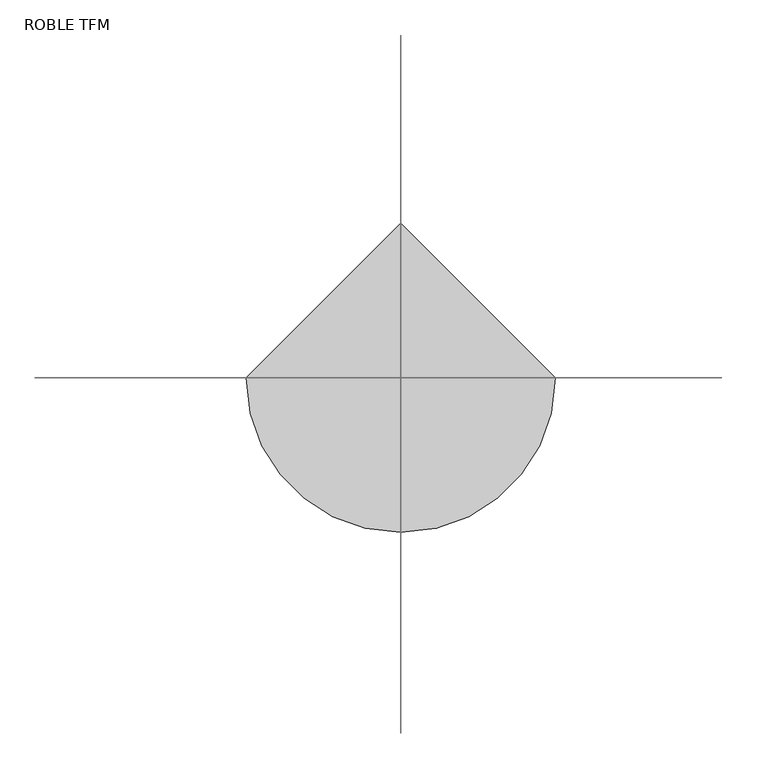
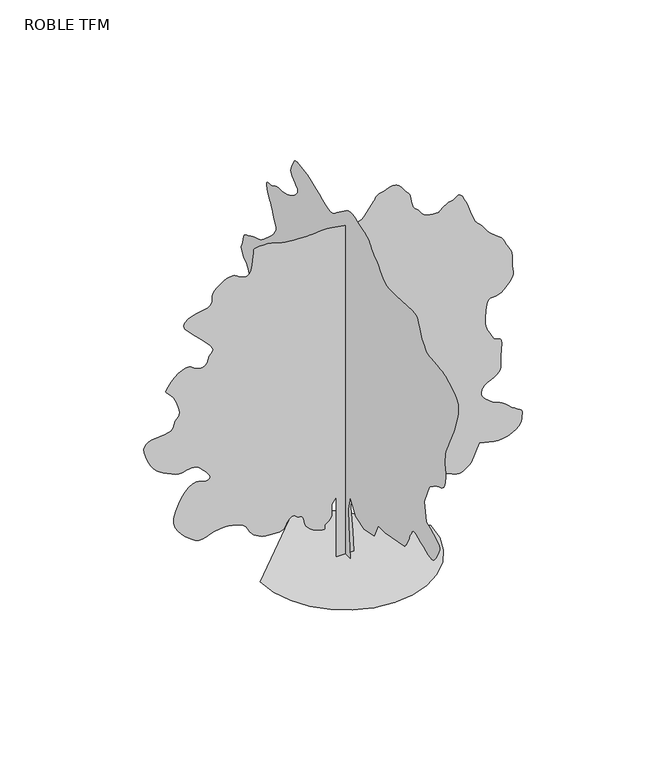
"""IFC4 building model written with IfcOpenShell, lengths in millimetres: geographic element geometry, RPC Árbol - Caducifolio : ROBLE TFM."""

from ifc_helpers import new_model, si_unit, origin, place, context, project, spatial, triangles, source, transform, mapped, element, save


def roble_tfm_b0279198(model_context):
    return source(origin(), model_context, "Body", "Tessellation", [
        triangles([(0.0082802, 146.8836034, 0.0), (0.0082802, -140.9112027, 0.0), (0.0082802, -94.4927969, 547.737606), (0.0082802, -85.2088796, 807.6804239), (0.0082802, -140.9112027, 1049.0568243), (0.0082802, -289.4507915, 807.6804239), (0.0082802, -530.8259929, 733.4111927), (0.0082802, -809.3364275, 798.397197), (0.0082802, -920.7408194, 1030.4892076), (0.0082802, -1115.6988321, 1030.4892076), (0.0082802, -1654.1519394, 1132.6103725), (0.0082802, -1673.9639568, 1156.5095678), (0.0082802, -1693.2960617, 1180.5708172), (0.0082802, -1711.6440697, 1204.9560293), (0.0082802, -1728.5280682, 1229.8320545), (0.0082802, -1743.4679993, 1255.3559326), (0.0082802, -1755.9720325, 1281.69604), (0.0082802, -1765.5599648, 1308.9959724), (0.0082802, -1774.8720417, 1337.124052), (0.0082802, -1786.6200165, 1365.7320442), (0.0082802, -1800.3960651, 1394.7480057), (0.0082802, -1815.7919277, 1424.0879299), (0.0082802, -1832.4119888, 1453.6679558), (0.0082802, -1849.8360706, 1483.4159946), (0.0082802, -1867.6800396, 1513.2359768), (0.0082802, -1876.1760326, 1522.8720165), (0.0082802, -1887.9240074, 1530.6479954), (0.0082802, -1906.1640278, 1534.6800167), (0.0082802, -1934.1479301, 1533.1080196), (0.0082802, -1975.1279869, 1524.0719433), (0.0082802, -2032.3439713, 1505.6880363), (0.0082802, -2109.0480103, 1476.1080105), (0.0082802, -2190.0359447, 1441.2960365), (0.0082802, -2259.0000492, 1410.2280201), (0.0082802, -2317.5720554, 1385.4840363), (0.0082802, -2367.372068, 1369.6800591), (0.0082802, -2410.0319641, 1365.4079361), (0.0082802, -2447.1599304, 1375.259951), (0.0082802, -2480.4000526, 1401.8400146), (0.0082802, -2513.9398659, 1443.7079533), (0.0082802, -2548.6080986, 1494.6719936), (0.0082802, -2581.0078651, 1550.1840122), (0.0082802, -2607.7198975, 1605.6960308), (0.0082802, -2625.3359734, 1656.6600712), (0.0082802, -2630.4600792, 1698.5399277), (0.0082802, -2619.6598663, 1726.7639317), (0.0082802, -2593.2719421, 1748.0159775), (0.0082802, -2555.18386, 1771.6920033), (0.0082802, -2507.3641045, 1797.4080208), (0.0082802, -2451.7320351, 1824.7439976), (0.0082802, -2390.2680542, 1853.3040276), (0.0082802, -2324.9040207, 1882.6679329), (0.0082802, -2257.5960651, 1912.4399529), (0.0082802, -2201.8920525, 2228.0879826), (0.0082802, -2341.1399483, 2553.0118996), (0.0082802, -2345.5319767, 2559.2158813), (0.0082802, -2352.3479851, 2566.7880936), (0.0082802, -2364.0479977, 2577.1319389), (0.0082802, -2383.0439312, 2591.6159386), (0.0082802, -2411.7840374, 2611.6080322), (0.0082802, -2452.7159866, 2638.5119133), (0.0082802, -2508.2521317, 2673.7080208), (0.0082802, -2568.5039772, 2705.5921211), (0.0082802, -2621.9280418, 2726.4239891), (0.0082802, -2668.5359528, 2743.368013), (0.0082802, -2708.3280006, 2763.5638733), (0.0082802, -2741.2919769, 2794.1521225), (0.0082802, -2767.4400902, 2842.2718597), (0.0082802, -2786.7601318, 2915.0761368), (0.0082802, -2797.9440422, 2986.5839813), (0.0082802, -2801.160125, 3032.4361244), (0.0082802, -2798.7001007, 3062.2081444), (0.0082802, -2792.8199364, 3085.4881187), (0.0082802, -2785.8119339, 3111.8519165), (0.0082802, -2779.9439781, 3150.875988), (0.0082802, -2777.4839539, 3212.160038), (0.0082802, -2778.3481453, 3279.7681206), (0.0082802, -2782.140065, 3335.8440582), (0.0082802, -2790.636058, 3387.0601181), (0.0082802, -2805.6240967, 3440.0519417), (0.0082802, -2828.904071, 3501.4920868), (0.0082802, -2862.2520355, 3578.0400307), (0.0082802, -2907.4440445, 3676.343914), (0.0082802, -2950.3559601, 3765.2038971), (0.0082802, -2978.9640976, 3818.8201012), (0.0082802, -2998.307975, 3851.9759262), (0.0082802, -3013.4399002, 3879.444017), (0.0082802, -3029.3880547, 3916.0080643), (0.0082802, -3051.1681206, 3976.4520493), (0.0082802, -3083.8440331, 4075.5361176), (0.0082802, -3119.0520584, 4190.159935), (0.0082802, -3142.7398567, 4288.871933), (0.0082802, -3151.3198563, 4373.9399963), (0.0082802, -3141.2161125, 4447.6439278), (0.0082802, -3108.8759354, 4512.2519028), (0.0082802, -3050.7120438, 4570.0320969), (0.0082802, -2963.1479118, 4623.2759399), (0.0082802, -2878.1879814, 4667.0401291), (0.0082802, -2822.3038925, 4697.1720108), (0.0082802, -2783.6280556, 4717.0559715), (0.0082802, -2750.3039268, 4730.1359871), (0.0082802, -2710.4880432, 4739.7958626), (0.0082802, -2652.3238609, 4749.4560287), (0.0082802, -2563.955999, 4762.5360443), (0.0082802, -2469.1678894, 4772.844136), (0.0082802, -2395.6559521, 4776.8279045), (0.0082802, -2337.408054, 4781.7720795), (0.0082802, -2288.4239799, 4795.0078995), (0.0082802, -2242.6799698, 4823.8320122), (0.0082802, -2194.1759537, 4875.5640289), (0.0082802, -2136.8999439, 4957.4880981), (0.0082802, -2086.8839561, 5047.5599258), (0.0082802, -2057.3280567, 5119.9438797), (0.0082802, -2038.0080151, 5176.2357925), (0.0082802, -2018.6760555, 5218.0797501), (0.0082802, -1989.1200108, 5247.0960022), (0.0082802, -1939.104023, 5264.9042175), (0.0082802, -1858.3919437, 5273.1362732), (0.0082802, -1412.7720509, 5245.2839035), (0.0082802, -1330.6320065, 5246.7239319), (0.0082802, -1263.7560013, 5246.5320831), (0.0082802, -1206.9359957, 5249.9161789), (0.0082802, -1154.9975962, 5262.0602051), (0.0082802, -1102.7328358, 5288.1841919), (0.0082802, -1044.9468281, 5333.4599167), (0.0082802, -976.4424339, 5403.107991), (0.0082802, -910.4291668, 5473.4519531), (0.0082802, -860.9784061, 5521.3798416), (0.0082802, -824.1959856, 5552.9162888), (0.0082802, -796.1819979, 5574.0597656), (0.0082802, -773.0411865, 5590.8122314), (0.0082802, -750.8735716, 5609.1837845), (0.0082802, -725.7839693, 5635.2002197), (0.0082802, -701.695178, 5665.9198563), (0.0082802, -681.9899855, 5694.5279938), (0.0082802, -661.9619928, 5721.1920639), (0.0082802, -636.8987698, 5746.0562439), (0.0082802, -602.091592, 5769.3118011), (0.0082802, -552.830391, 5791.1040756), (0.0082802, -484.4076053, 5811.5882904), (0.0082802, -407.594416, 5834.1601685), (0.0082802, -335.9772031, 5859.1679443), (0.0082802, -269.0688053, 5882.2322342), (0.0082802, -206.3844047, 5898.9602829), (0.0082802, -147.4343965, 5904.9721252), (0.0082802, -91.7318372, 5895.8761688), (0.0082802, -38.7904784, 5867.2918671), (0.0082802, 239.7203968, 5663.0520081), (0.0082802, 269.8716087, 5635.607753), (0.0082802, 299.0496061, 5610.5999771), (0.0082802, 330.8243926, 5590.4517883), (0.0082802, 368.7720037, 5577.6240829), (0.0082802, 416.4624066, 5574.5399689), (0.0082802, 477.4691843, 5583.6359253), (0.0082802, 555.3659921, 5607.34785), (0.0082802, 643.7639757, 5642.5561661), (0.0082802, 732.8112293, 5682.1560745), (0.0082802, 820.8839785, 5722.5722122), (0.0082802, 906.3587757, 5760.2158447), (0.0082802, 987.6120283, 5791.536026), (0.0082802, 1063.0176001, 5812.9440216), (0.0082802, 1130.954369, 5820.8760956), (0.0082802, 1192.7460188, 5825.2078079), (0.0082802, 1250.1479656, 5835.0601135), (0.0082802, 1302.2039452, 5845.7158585), (0.0082802, 1347.9120564, 5852.48405), (0.0082802, 1386.3239559, 5850.6481155), (0.0082802, 1416.4440651, 5835.4920639), (0.0082802, 1437.3119774, 5802.2999039), (0.0082802, 1455.959967, 5760.6001236), (0.0082802, 1477.3679626, 5722.1402618), (0.0082802, 1497.4799618, 5685.6238861), (0.0082802, 1512.239962, 5649.7557266), (0.0082802, 1517.5679798, 5613.2521408), (0.0082802, 1509.4199306, 5574.7922791), (0.0082802, 1483.7399574, 5533.0802902), (0.0082802, 1444.4400307, 5494.8599487), (0.0082802, 1402.3680347, 5464.9199158), (0.0082802, 1363.8840466, 5439.0482391), (0.0082802, 1335.3000355, 5413.0079681), (0.0082802, 1322.9640152, 5382.5877319), (0.0082802, 1333.1879551, 5343.5639511), (0.0082802, 1372.3319321, 5291.7002563), (0.0082802, 1426.3799412, 5240.027829), (0.0082802, 1477.3439816, 5202.3359436), (0.0082802, 1525.548016, 5175.5038605), (0.0082802, 1571.3160072, 5156.4840912), (0.0082802, 1614.9720634, 5142.155896), (0.0082802, 1656.8520653, 5129.4717865), (0.0082802, 1697.2559944, 5115.3121857), (0.0082802, 1737.6119614, 5104.4041306), (0.0082802, 1779.107975, 5100.8037689), (0.0082802, 1821.7319721, 5100.4561157), (0.0082802, 1865.4960159, 5099.2922333), (0.0082802, 1910.3999611, 5093.2559738), (0.0082802, 1956.4439529, 5078.2801437), (0.0082802, 2003.6159283, 5050.3318497), (0.0082802, 2052.3719639, 5025.503714), (0.0082802, 2100.2999977, 5016.6001877), (0.0082802, 2143.1999954, 5014.5119431), (0.0082802, 2176.8479416, 5010.1558136), (0.0082802, 2197.0080482, 4994.4358429), (0.0082802, 2199.4680725, 4958.243866), (0.0082802, 2180.0160622, 4892.5077621), (0.0082802, 2151.2640381, 4823.3279732), (0.0082802, 2127.3960182, 4776.7200623), (0.0082802, 2106.4439541, 4743.42006), (0.0082802, 2086.4759869, 4714.1881233), (0.0082802, 2065.5240681, 4679.7599922), (0.0082802, 2041.643985, 4630.8839058), (0.0082802, 2012.9040241, 4558.2958946), (0.0082802, 1982.5320408, 4486.8958923), (0.0082802, 1956.3959908, 4441.8000984), (0.0082802, 1936.4159603, 4414.0799881), (0.0082802, 1924.5599979, 4394.8079086), (0.0082802, 1922.7720257, 4375.0559166), (0.0082802, 1933.0080288, 4345.8719421), (0.0082802, 1957.2000114, 4298.3518776), (0.0082802, 2000.2680222, 4235.3638618), (0.0082802, 2060.6999439, 4168.488002), (0.0082802, 2130.8879562, 4101.7679466), (0.0082802, 2203.1759857, 4039.272052), (0.0082802, 2269.9560665, 3985.0558846), (0.0082802, 2323.5719799, 3943.1880913), (0.0082802, 2356.4039875, 3917.71203), (0.0082802, 2385.552063, 3901.7760841), (0.0082802, 2429.3159615, 3885.6721252), (0.0082802, 2481.8519989, 3869.2440582), (0.0082802, 2537.3160553, 3852.3238701), (0.0082802, 2589.8520927, 3834.7560471), (0.0082802, 2633.6159912, 3816.3839127), (0.0082802, 2662.7639214, 3797.0281174), (0.0082802, 2687.1720245, 3780.9479942), (0.0082802, 2718.2521042, 3769.5838623), (0.0082802, 2752.4040894, 3758.5441292), (0.0082802, 2786.0758713, 3743.4360397), (0.0082802, 2815.6920868, 3719.892128), (0.0082802, 2837.6640015, 3683.5080116), (0.0082802, 2848.4400879, 3629.915934), (0.0082802, 2857.2598984, 3576.0840454), (0.0082802, 2872.41595, 3538.0078812), (0.0082802, 2888.8681435, 3509.8319847), (0.0082802, 2901.5999245, 3485.7119453), (0.0082802, 2905.5479393, 3459.8161423), (0.0082802, 2895.6959244, 3426.2760384), (0.0082802, 2867.004071, 3379.2600128), (0.0082802, 2831.3879311, 3335.2199684), (0.0082802, 2802.5879448, 3308.8919243), (0.0082802, 2778.3359367, 3291.8159317), (0.0082802, 2756.3521042, 3275.5439598), (0.0082802, 2734.3798988, 3251.6398956), (0.0082802, 2710.1278908, 3211.6679169), (0.0082802, 2681.3279045, 3147.1680748), (0.0082802, 2649.9359253, 3082.5600998), (0.0082802, 2621.135939, 3041.8320625), (0.0082802, 2597.5318565, 3015.8760887), (0.0082802, 2581.7278793, 2995.5959312), (0.0082802, 2576.3160004, 2971.9200508), (0.0082802, 2583.8879219, 2935.7280739), (0.0082802, 2607.060054, 2877.9478798), (0.0082802, 2637.8398613, 2814.7438889), (0.0082802, 2666.8200691, 2765.6759537), (0.0082802, 2694.516053, 2726.6760086), (0.0082802, 2721.3838898, 2693.675988), (0.0082802, 2747.9401176, 2662.6319527), (0.0082802, 2774.6518593, 2629.4761276), (0.0082802, 2802.0121078, 2590.1520744), (0.0082802, 2833.7639488, 2551.3681046), (0.0082802, 2870.7119843, 2519.7241058), (0.0082802, 2908.9558708, 2491.0081261), (0.0082802, 2944.6080551, 2460.9840866), (0.0082802, 2973.7559853, 2425.4519531), (0.0082802, 2992.5121078, 2380.1640198), (0.0082802, 2996.9760796, 2320.9199615), (0.0082802, 3000.731955, 2274.3960571), (0.0082802, 3014.568029, 2259.0480114), (0.0082802, 3030.3478798, 2258.315934), (0.0082802, 3039.9600838, 2255.6399345), (0.0082802, 3035.2679283, 2234.4480595), (0.0082802, 3008.1841164, 2178.1799824), (0.0082802, 2950.5600174, 2070.2640404), (0.0082802, 2890.3078812, 1949.2199753), (0.0082802, 2853.9359734, 1860.1800613), (0.0082802, 2831.1960823, 1796.4599682), (0.0082802, 2811.8760406, 1751.4240543), (0.0082802, 2785.7279274, 1718.4000526), (0.0082802, 2742.527948, 1690.7399677), (0.0082802, 2672.0520172, 1661.7840317), (0.0082802, 2590.6799492, 1638.2879368), (0.0082802, 2519.0639717, 1628.4360672), (0.0082802, 2453.2921143, 1627.6800087), (0.0082802, 2389.4759514, 1631.4719284), (0.0082802, 2323.7039486, 1635.2519302), (0.0082802, 2252.0879711, 1634.4960171), (0.0082802, 2170.7279663, 1624.6440022), (0.0082802, 2089.5839367, 1615.8240463), (0.0082802, 2019.4799309, 1617.7200062), (0.0082802, 1957.8239559, 1625.1359779), (0.0082802, 1902.0119556, 1632.8760578), (0.0082802, 1849.4519371, 1635.7440514), (0.0082802, 1797.5399895, 1628.5440548), (0.0082802, 1743.6720566, 1606.080019), (0.0082802, 1692.1199707, 1582.1999359), (0.0082802, 1649.4840557, 1569.696048), (0.0082802, 1616.7600357, 1561.7399929), (0.0082802, 1594.9199444, 1551.516053), (0.0082802, 1584.9359608, 1532.1839481), (0.0082802, 1587.7799732, 1496.9519417), (0.0082802, 1604.4240154, 1438.967981), (0.0082802, 1631.2680164, 1377.3720314), (0.0082802, 1663.4759342, 1333.7880638), (0.0082802, 1700.1600323, 1305.2399517), (0.0082802, 1740.4080116, 1288.7040424), (0.0082802, 1783.3319904, 1281.1799377), (0.0082802, 1828.0439415, 1279.6560482), (0.0082802, 1873.6440651, 1281.1440388), (0.0082802, 2050.0440536, 1086.1919849), (0.0082802, 2063.8680645, 1064.2404179), (0.0082802, 2077.1280109, 1041.8843697), (0.0082802, 2089.2599739, 1018.7160164), (0.0082802, 2099.6760532, 994.3284061), (0.0082802, 2107.8239571, 968.3183659), (0.0082802, 2113.1279938, 940.2779989), (0.0082802, 2115.0239536, 909.8015888), (0.0082802, 2114.6999908, 878.0256214), (0.0082802, 2112.4319607, 846.5747795), (0.0082802, 2106.25196, 815.7744066), (0.0082802, 2094.2400478, 785.9472301), (0.0082802, 2074.4280304, 757.419611), (0.0082802, 2044.8719856, 730.5155846), (0.0082802, 2003.6159283, 705.5604218), (0.0082802, 1964.2680393, 684.3671659), (0.0082802, 1936.6079544, 667.8840151), (0.0082802, 1913.0040173, 655.136392), (0.0082802, 1885.8239902, 645.1487749), (0.0082802, 1847.4479897, 636.9479673), (0.0082802, 1790.2320053, 629.5583748), (0.0082802, 1706.5439449, 622.0068008), (0.0082802, 1611.3480114, 623.0892202), (0.0082802, 1523.6279297, 639.7619671), (0.0082802, 1441.751968, 668.2908216), (0.0082802, 1364.1000217, 704.9375673), (0.0082802, 1289.0519863, 745.9703825), (0.0082802, 1214.963994, 787.6524313), (0.0082802, 1140.2375959, 826.2479679), (0.0082802, 1073.6003843, 861.3528019), (0.0082802, 1022.0663933, 894.5087723), (0.0082802, 981.4127701, 924.9048094), (0.0082802, 947.4179701, 951.7272274), (0.0082802, 915.8592133, 974.1648113), (0.0082802, 882.5135742, 991.4064188), (0.0082802, 843.159581, 1002.638364), (0.0082802, 799.8803913, 1012.111187), (0.0082802, 757.251598, 1023.857999), (0.0082802, 714.784786, 1036.742387), (0.0082802, 671.9940113, 1049.6256123), (0.0082802, 628.3896235, 1061.3724243), (0.0082802, 583.4868047, 1070.8451746), (0.0082802, 536.7984118, 1076.9075953), (0.0082802, 489.054015, 1080.0744078), (0.0082802, 441.3083828, 1081.7796089), (0.0082802, 393.563986, 1082.2667885), (0.0082802, 345.8195892, 1081.7796089), (0.0082802, 298.0751925, 1080.5615873), (0.0082802, 250.3295966, 1078.8563862), (0.0082802, 202.5851998, 1076.9075953), (0.0082802, 109.7486426, 937.6524324), (0.0082802, 91.1810441, 724.1279657), (134.6136038, 0.0002884, 0.0044219), (-143.8968035, 0.0002884, 0.0044219), (-143.8968035, 0.0002283, 1021.2096142), (-218.1672066, 0.0002283, 919.089612), (-218.1672066, 0.0002403, 807.6852201), (-216.4620054, 0.0002403, 781.8372339), (-216.4620054, 0.0002403, 756.0696207), (-219.8724077, 0.0002403, 730.4652243), (-228.3971962, 0.0002523, 705.1044176), (-243.7440066, 0.0002523, 680.0688091), (-267.6168045, 0.0002523, 655.4376091), (-301.7195921, 0.0002523, 631.294824), (-328.4339862, 0.0002523, 606.231601), (-335.8236151, 0.0002523, 580.843216), (-334.1184139, 0.0002523, 558.2171988), (-333.5495896, 0.0002523, 541.4351927), (-344.3495845, 0.0002523, 533.5859988), (-376.7472073, 0.0002523, 537.7547851), (-440.9747912, 0.0002523, 557.0255928), (-514.2432115, 0.0002523, 587.0424016), (-568.9980088, 0.0002523, 620.9556295), (-608.3243875, 0.0002523, 658.1184048), (-635.3099859, 0.0002523, 697.8779692), (-653.038773, 0.0002403, 739.5863972), (-664.595989, 0.0002403, 782.5943825), (-673.068001, 0.0002403, 826.2527641), (-675.2327671, 0.0002403, 838.1340157), (-678.4535734, 0.0002403, 849.6912317), (-683.7852247, 0.0002403, 860.6003769), (-692.2847786, 0.0002403, 870.5327648), (-705.0047871, 0.0002403, 879.1668308), (-723.0047785, 0.0002403, 886.1772314), (-747.3372322, 0.0002403, 891.2387684), (-771.6696133, 0.0002403, 899.5740154), (-790.8047825, 0.0002403, 913.5948166), (-807.5052166, 0.0002283, 928.7520309), (-824.5296135, 0.0002283, 940.4987703), (-844.6403772, 0.0002283, 944.2883646), (-870.5964237, 0.0002283, 935.5728355), (-905.1600117, 0.0002403, 909.8052223), (-935.5548134, 0.0002403, 873.7535711), (-952.7964209, 0.0002403, 838.5132076), (-965.3279961, 0.0002403, 806.0340128), (-981.594009, 0.0002403, 778.2636148), (-1010.0411825, 0.0002403, 757.1532028), (-1059.1115885, 0.0002403, 744.6480068), (-1137.2520224, 0.0002403, 742.6992159), (-1223.5920284, 0.0002403, 748.4376011), (-1293.6960342, 0.0002403, 757.910424), (-1350.636018, 0.0002403, 771.443973), (-1397.5199295, 0.0002403, 789.3611933), (-1437.419965, 0.0002403, 811.9883732), (-1473.4080299, 0.0002403, 839.6507835), (-1508.6039921, 0.0002403, 872.6712244), (-1538.4479553, 0.0002403, 908.8847843), (-1559.8680141, 0.0002283, 945.2627964), (-1578.024028, 0.0002283, 980.8271954), (-1598.1360271, 0.0002283, 1014.6060202), (-1625.3879974, 0.0002283, 1045.6236036), (-1664.9880512, 0.0002283, 1072.906822), (-1722.1200291, 0.0002283, 1095.4800081), (-1779.5640518, 0.0002283, 1112.6387718), (-1821.2399963, 0.0002163, 1124.7647758), (-1854.1560104, 0.0002163, 1132.5060184), (-1885.2840523, 0.0002163, 1136.5115879), (-1921.5959347, 0.0002163, 1137.4320259), (-1970.0999508, 0.0002163, 1135.9164207), (-2037.7680588, 0.0002163, 1132.614006), (-2112.1680233, 0.0002163, 1120.8948086), (-2178.3000332, 0.0002283, 1099.1063856), (-2239.2239307, 0.0002283, 1075.3691717), (-2298.0360386, 0.0002283, 1057.8036015), (-2357.8319527, 0.0002283, 1054.5288013), (-2421.6719513, 0.0002283, 1073.6639706), (-2492.6641296, 0.0002163, 1123.3307791), (-2566.943898, 0.0002163, 1189.7507801), (-2635.5240143, 0.0002163, 1255.6800407), (-2693.8800453, 0.0002043, 1324.0559544), (-2737.452095, 0.0002043, 1397.7840122), (-2761.7041031, 0.0002043, 1479.7919426), (-2762.0880913, 0.0001923, 1573.0080551), (-2734.0438728, 0.0001923, 1680.3480148), (-2687.1121445, 0.0001802, 1788.6120461), (-2634.815918, 0.0001802, 1881.4559429), (-2578.6321381, 0.0001682, 1957.0799606), (-2520.011879, 0.0001682, 2013.6959816), (-2460.407959, 0.0001682, 2049.5279514), (-2401.2960148, 0.0001682, 2062.7999611), (-2344.1279926, 0.0001682, 2051.7000572), (-2290.2119522, 0.0001682, 2033.0279411), (-2242.4760578, 0.0001682, 2025.0599682), (-2204.795945, 0.0001682, 2028.3119499), (-2181.0840202, 0.0001682, 2043.2520264), (-2175.2400455, 0.0001682, 2070.372028), (-2191.1520103, 0.0001682, 2110.1639305), (-2232.7199673, 0.0001562, 2163.1079372), (-2281.2000023, 0.0001562, 2216.2080391), (-2318.1480377, 0.0001562, 2257.1280704), (-2347.9440388, 0.0001562, 2287.3320408), (-2374.9800339, 0.0001562, 2308.2839596), (-2403.6480515, 0.0001562, 2321.4360638), (-2438.3159935, 0.0001442, 2328.26399), (-2483.3879517, 0.0001442, 2330.2080574), (-2529.6118744, 0.0001562, 2325.8519279), (-2567.8920959, 0.0001562, 2315.8080643), (-2602.7518867, 0.0001562, 2304.6360718), (-2638.7520149, 0.0001562, 2296.8599476), (-2680.4279594, 0.0001562, 2297.0519417), (-2732.3399071, 0.0001562, 2309.7479691), (-2799.0361267, 0.0001442, 2339.4960079), (-2869.8120392, 0.0001442, 2375.0880215), (-2932.1399208, 0.0001442, 2405.9640438), (-2987.8199524, 0.0001442, 2437.6680679), (-3038.6159798, 0.0001442, 2475.6959793), (-3086.3401016, 0.0001442, 2525.5679352), (-3132.7558731, 0.0001322, 2592.8280739), (-3179.6640564, 0.0001322, 2682.9961166), (-3218.4480263, 0.0001202, 2776.5598824), (-3239.8560219, 0.0001202, 2851.7759308), (-3244.7039818, 0.0001202, 2910.7560516), (-3233.7959267, 0.0001081, 2955.6001167), (-3207.9480858, 0.0001081, 2988.4321243), (-3167.976107, 0.0001081, 3011.3519463), (-3114.6720932, 0.0001081, 3026.4838715), (-3051.7439575, 0.0001081, 3035.1720039), (-2985.2520859, 0.0001081, 3040.2961098), (-2919.5520264, 0.0001081, 3046.2120277), (-2859.0600792, 0.0001081, 3057.336058), (-2808.1559189, 0.0001081, 3078.0478752), (-2771.2078835, 0.0001081, 3112.7161079), (-2752.607856, 9.61e-05, 3165.7439758), (-2738.867997, 9.61e-05, 3216.9481178), (-2717.6399323, 9.61e-05, 3250.2960823), (-2695.1279343, 9.61e-05, 3276.3360626), (-2677.4761047, 9.61e-05, 3305.6159615), (-2670.8759262, 8.41e-05, 3348.7080986), (-2681.4839996, 8.41e-05, 3416.1600861), (-2715.4798897, 8.41e-05, 3518.5201172), (-2763.624044, 7.21e-05, 3619.3439049), (-2809.6680359, 7.21e-05, 3682.8121239), (-2849.2080643, 7.21e-05, 3720.4679649), (-2877.8760818, 6.01e-05, 3743.8200279), (-2891.267997, 6.01e-05, 3764.412085), (-2885.016053, 6.01e-05, 3793.7879082), (-2854.7280762, 6.01e-05, 3843.4560974), (-2805.9118698, 6.01e-05, 3905.4360352), (-2749.451944, 4.81e-05, 3961.895961), (-2689.0919655, 4.81e-05, 4009.5840385), (-2628.563974, 4.81e-05, 4045.2600586), (-2571.6241356, 4.81e-05, 4065.6599762), (-2521.9800728, 4.81e-05, 4067.5560814), (-2483.3879517, 4.81e-05, 4047.6959564), (-2445.551889, 4.81e-05, 4018.0800316), (-2398.9439781, 4.81e-05, 3994.9680702), (-2348.4360146, 4.81e-05, 3981.4319778), (-2298.8999393, 4.81e-05, 3980.5680771), (-2255.2200474, 4.81e-05, 3995.4599007), (-2222.2560711, 4.81e-05, 4029.1799355), (-2204.8799515, 4.81e-05, 4084.8239227), (-2188.9560688, 4.81e-05, 4137.8759171), (-2163.9480022, 3.6e-05, 4169.328067), (-2140.0799824, 3.6e-05, 4190.5439232), (-2127.5759491, 3.6e-05, 4212.9001167), (-2136.6720509, 3.6e-05, 4247.7599075), (-2177.5919369, 3.6e-05, 4306.4999268), (-2260.5839642, 2.4e-05, 4400.4720978), (-2364.647961, 2.4e-05, 4506.6240486), (-2457.6720795, 1.2e-05, 4596.0479507), (-2533.1639832, 1.2e-05, 4671.3480057), (-2584.6079361, 1.2e-05, 4735.1159157), (-2605.5360191, 0.0, 4789.9558823), (-2589.4320602, 0.0, 4838.4598984), (-2529.8040138, 0.0, 4883.219957), (-2450.2800888, 0.0, 4917.7079681), (-2379.0479542, 0.0, 4937.411998), (-2316.4199455, 0.0, 4948.0200714), (-2262.7200256, -1.2e-05, 4955.2202133), (-2218.2720119, -1.2e-05, 4964.6882401), (-2183.4119305, -1.2e-05, 4982.1238037), (-2158.4519714, -1.2e-05, 5013.1922562), (-2146.0079636, -1.2e-05, 5049.9481522), (-2144.1120037, -1.2e-05, 5082.1560699), (-2146.2720463, -1.2e-05, 5112.0961029), (-2146.0079636, -1.2e-05, 5142.0361359), (-2136.8040195, -2.4e-05, 5174.2440536), (-2112.1680233, -2.4e-05, 5210.9999496), (-2065.6199924, -2.4e-05, 5254.57229), (-2008.6439644, -2.4e-05, 5297.6882629), (-1956.5400227, -2.4e-05, 5331.2280762), (-1908.5040012, -3.6e-05, 5354.6882721), (-1863.7080437, -3.6e-05, 5367.6002747), (-1821.3479839, -3.6e-05, 5369.4722534), (-1780.6080288, -3.6e-05, 5359.8001694), (-1740.6959301, -2.4e-05, 5338.1282364), (-1699.5480057, -2.4e-05, 5311.6321793), (-1657.1160027, -2.4e-05, 5290.9799515), (-1615.4880203, -2.4e-05, 5280.8759171), (-1576.7759937, -2.4e-05, 5286.0482758), (-1543.1040665, -2.4e-05, 5311.1880203), (-1516.5840282, -3.6e-05, 5361.0239319), (-1499.3160416, -3.6e-05, 5440.2481659), (-1489.0079498, -3.6e-05, 5525.3162292), (-1481.6159592, -4.81e-05, 5591.0517517), (-1476.6600117, -4.81e-05, 5639.7481979), (-1473.6600494, -4.81e-05, 5673.6600815), (-1472.1120335, -4.81e-05, 5695.0680771), (-1471.5479691, -4.81e-05, 5706.2522781), (-1471.4639626, -4.81e-05, 5709.4677795), (-1459.2600563, -4.81e-05, 5711.3641754), (-1426.1039406, -4.81e-05, 5715.5400833), (-1377.1919552, -4.81e-05, 5719.7037827), (-1317.7320671, -4.81e-05, 5721.6001785), (-1252.9079716, -4.81e-05, 5718.9480148), (-1187.9195692, -4.81e-05, 5709.4677795), (-1127.9687954, -4.81e-05, 5690.9037964), (-1072.9967875, -4.81e-05, 5670.25215), (-1017.8627981, -4.81e-05, 5655.2879471), (-960.1307842, -4.81e-05, 5644.8600952), (-897.3636126, -4.81e-05, 5637.8518021), (-827.1275654, -4.81e-05, 5633.1241837), (-746.9844194, -4.81e-05, 5629.523822), (-654.4992216, -4.81e-05, 5625.9240417), (-565.2359928, -4.81e-05, 5625.4077942), (-491.7239828, -4.81e-05, 5629.7639236), (-426.9816047, -4.81e-05, 5635.9077347), (-364.0259997, -4.81e-05, 5640.7562759), (-295.8744002, -4.81e-05, 5641.2120621), (-215.5416038, -4.81e-05, 5634.2037689), (-116.0463596, -4.81e-05, 5616.6362366), (-15.46836, -4.81e-05, 5595.7439072), (65.6219983, -4.81e-05, 5581.3442047), (130.4723958, -4.81e-05, 5574.2521957), (182.3316032, -4.81e-05, 5575.2719009), (224.4468015, -4.81e-05, 5585.2439667), (260.0651942, -4.81e-05, 5604.9479965), (292.4364015, -4.81e-05, 5635.2002197), (431.6916006, -6.01e-05, 5811.5882904), (452.5872002, -6.01e-05, 5838.7918625), (469.2599833, -6.01e-05, 5864.375766), (484.3080111, -6.01e-05, 5887.8359619), (500.3315969, -6.01e-05, 5908.7038742), (519.9276029, -6.01e-05, 5926.4882538), (545.6952161, -6.01e-05, 5940.6961075), (580.2311894, -6.01e-05, 5950.8478134), (622.5624355, -7.21e-05, 5962.4878006), (668.7912271, -7.21e-05, 5978.0281311), (717.1307911, -7.21e-05, 5992.2598206), (765.7967886, -7.21e-05, 6000.0000458), (813.000012, -7.21e-05, 5996.0520309), (856.9548145, -7.21e-05, 5975.2079544), (895.8767847, -6.01e-05, 5932.2838303), (930.4392099, -6.01e-05, 5883.324028), (962.0795752, -6.01e-05, 5845.2362366), (990.1476294, -6.01e-05, 5814.1317398), (1013.9928308, -6.01e-05, 5786.124147), (1032.9660187, -6.01e-05, 5757.2997437), (1046.4180319, -4.81e-05, 5723.7599304), (1053.6984015, -4.81e-05, 5681.6159912), (1058.7600111, -4.81e-05, 5637.9360992), (1065.7704117, -4.81e-05, 5601.5639008), (1074.404405, -4.81e-05, 5571.2762146), (1084.3367929, -3.6e-05, 5545.8597427), (1095.2447754, -3.6e-05, 5524.0918854), (1106.8019915, -3.6e-05, 5504.7721344), (1118.6844057, -3.6e-05, 5486.6639374), (1130.7011868, -3.6e-05, 5478.5161789), (1143.2063828, -3.6e-05, 5469.2277924), (1156.6847752, -3.6e-05, 5457.6721024), (1171.6260143, -3.6e-05, 5442.7078995), (1188.514809, -3.6e-05, 5423.1957184), (1207.8360134, -3.6e-05, 5397.9960938), (1230.0839287, -3.6e-05, 5365.9800247), (1263.0599682, -2.4e-05, 5335.5481613), (1309.6680244, -2.4e-05, 5314.715712), (1363.0919437, -2.4e-05, 5301.6601135), (1416.5160084, -2.4e-05, 5294.6279846), (1463.1240646, -2.4e-05, 5291.8078079), (1496.0999588, -2.4e-05, 5291.4357376), (1508.6039921, -2.4e-05, 5291.7118835), (1515.0120312, -2.4e-05, 5298.3957779), (1532.6400249, -2.4e-05, 5315.6278656), (1559.0279491, -2.4e-05, 5339.2078217), (1591.7519691, -3.6e-05, 5364.8882309), (1628.3639786, -3.6e-05, 5388.468187), (1666.4520607, -3.6e-05, 5405.7119019), (1703.5560459, -3.6e-05, 5412.3957962), (1736.8200039, -3.6e-05, 5420.544136), (1766.1840546, -3.6e-05, 5438.9162704), (1793.4479427, -3.6e-05, 5458.4278702), (1820.3759502, -3.6e-05, 5469.9957687), (1848.7679672, -3.6e-05, 5464.500174), (1880.4119659, -3.6e-05, 5432.8561752), (1917.0840008, -3.6e-05, 5365.9800247), (1951.6199741, -2.4e-05, 5287.404007), (1977.3839539, -2.4e-05, 5223.935788), (1996.9799961, -2.4e-05, 5171.3401611), (2012.9999485, -1.2e-05, 5125.4162201), (2028.0480125, -1.2e-05, 5081.9159683), (2044.7279537, -1.2e-05, 5036.6402435), (2065.6199924, -1.2e-05, 4985.3398865), (2087.0880135, 0.0, 4940.3280991), (2105.4600025, 0.0, 4911.7199615), (2123.3519337, 0.0, 4892.051976), (2143.3559452, 0.0, 4873.8359367), (2168.0640301, 0.0, 4849.6080551), (2200.0799538, 0.0, 4811.9039612), (2242.0080631, 0.0, 4753.2479485), (2293.6200291, 1.2e-05, 4687.9679214), (2350.271949, 1.2e-05, 4633.4041008), (2407.896048, 1.2e-05, 4586.6278862), (2462.4360329, 2.4e-05, 4544.7359665), (2509.8241287, 2.4e-05, 4504.7881142), (2546.0161057, 2.4e-05, 4463.8560196), (2566.943898, 2.4e-05, 4419.0360809), (2583.371965, 2.4e-05, 4375.080043), (2606.2920776, 3.6e-05, 4335.6719833), (2631.9841141, 3.6e-05, 4296.2639236), (2656.6919083, 3.6e-05, 4252.3078857), (2676.6959198, 3.6e-05, 4199.2681), (2688.2519005, 4.81e-05, 4132.5718803), (2687.6281013, 4.81e-05, 4047.6959564), (2686.356086, 4.81e-05, 3966.1201218), (2693.3640884, 6.01e-05, 3906.624044), (2701.0200165, 6.01e-05, 3860.6160965), (2701.7039864, 6.01e-05, 3819.4680267), (2687.76007, 6.01e-05, 3774.6001259), (2651.580011, 7.21e-05, 3717.371933), (2585.5078812, 7.21e-05, 3639.2040298), (2507.0998764, 7.21e-05, 3573.576059), (2439.0839699, 7.21e-05, 3547.236097), (2381.615966, 7.21e-05, 3541.5239456), (2334.8759411, 7.21e-05, 3537.7680702), (2299.0080723, 8.41e-05, 3517.2719376), (2274.1919998, 8.41e-05, 3461.3881393), (2260.5720463, 8.41e-05, 3351.4201424), (2255.4839848, 9.61e-05, 3229.727861), (2256.2519611, 9.61e-05, 3144.0839607), (2263.0079441, 0.0001081, 3083.9518753), (2275.955991, 0.0001081, 3038.7479485), (2295.2280704, 0.0001081, 2997.9359047), (2320.9920502, 0.0001081, 2950.9440056), (2353.4159431, 0.0001202, 2887.2359756), (2390.4119408, 0.0001202, 2831.83209), (2427.7439644, 0.0001202, 2806.631884), (2462.3040642, 0.0001202, 2796.3720451), (2491.0200439, 0.0001202, 2785.7880981), (2510.8080803, 0.0001202, 2759.6158585), (2518.5721413, 0.0001322, 2702.5800957), (2511.2400307, 0.0001322, 2599.4398796), (2501.2798828, 0.0001442, 2485.7279251), (2499.7561386, 0.0001442, 2402.5559669), (2501.495858, 0.0001442, 2342.9280659), (2501.2798828, 0.0001562, 2299.871973), (2493.9120186, 0.0001562, 2266.3920399), (2474.2079887, 0.0001562, 2235.5039543), (2436.9720348, 0.0001562, 2200.2360489), (2391.9839378, 0.0001562, 2167.1639397), (2352.1920353, 0.0001562, 2144.8080368), (2317.1159786, 0.0001562, 2129.1120472), (2286.2639374, 0.0001682, 2116.0080505), (2259.1439358, 0.0001682, 2101.4519623), (2235.2760612, 0.0001682, 2081.3639442), (2214.1559841, 0.0001682, 2051.7000572), (2197.3799732, 0.0001682, 2017.3559326), (2187.9000286, 0.0001682, 1984.9560207), (2187.3599453, 0.0001682, 1953.0479393), (2197.3799732, 0.0001802, 1920.1560516), (2219.5680084, 0.0001802, 1884.8400387), (2255.5679913, 0.0001802, 1845.6120552), (2307.0000263, 0.0001802, 1801.0439907), (2361.5039669, 0.0001802, 1761.9840202), (2407.7399529, 0.0001802, 1736.3999714), (2448.7679718, 0.0001923, 1718.4599327), (2487.6961189, 0.0001923, 1702.3080116), (2527.5840912, 0.0001923, 1682.0880249), (2571.5401291, 0.0001923, 1651.9559978), (2622.6361382, 0.0001923, 1606.080019), (2676.8880592, 0.0001923, 1558.6920685), (2726.9039017, 0.0001923, 1524.7800396), (2770.7520973, 0.0002043, 1499.6279411), (2806.4760796, 0.0002043, 1478.5440536), (2832.1320717, 0.0002043, 1456.8119499), (2845.7760063, 0.0002043, 1429.7159294), (2845.4518982, 0.0002043, 1392.5520641), (2840.1240257, 0.0002043, 1350.3600174), (2836.8960251, 0.0002163, 1310.7599636), (2831.0760315, 0.0002163, 1272.9480274), (2817.9480537, 0.0002163, 1236.1200428), (2792.8080185, 0.0002163, 1199.4408136), (2750.9399345, 0.0002163, 1162.1159843), (2687.6281013, 0.0002163, 1123.3307791), (2612.0280647, 0.0002283, 1091.9340036), (2536.439946, 0.0002283, 1075.6403761), (2460.8399094, 0.0002283, 1071.9323902), (2385.2400181, 0.0002283, 1078.2923944), (2309.6520447, 0.0002283, 1092.2039726), (2234.0520081, 0.0002283, 1111.1507813), (2158.4519714, 0.0002163, 1132.614006), (2028.4799629, 0.0002403, 844.8203808), (1996.6320522, 0.0002403, 817.2119642), (1964.6040653, 0.0002403, 791.0663944), (1932.2640335, 0.0002403, 767.8439747), (1899.4320259, 0.0002403, 749.0052263), (1865.9519474, 0.0002403, 736.0140135), (1831.6559303, 0.0002403, 730.3307848), (1796.3880249, 0.0002403, 733.4159889), (1767.648064, 0.0002403, 740.4252268), (1749.4560059, 0.0002403, 746.2992142), (1736.47206, 0.0002403, 752.1732016), (1723.3199558, 0.0002403, 759.1823668), (1704.6360672, 0.0002403, 768.4668291), (1675.0800224, 0.0002403, 781.1603857), (1629.2880501, 0.0002403, 798.4019932), (1569.6360226, 0.0002403, 823.4376017), (1504.4639832, 0.0002403, 856.593572), (1437.3359585, 0.0002403, 894.6216288), (1371.8399563, 0.0002283, 934.2732056), (1311.52794, 0.0002283, 972.3011896), (1259.9999805, 0.0002283, 1005.4572327), (1220.8080414, 0.0002283, 1030.4940039), (1187.6219856, 0.0002283, 1052.5523958), (1152.0035929, 0.0002283, 1078.5083696), (1114.3535654, 0.0002283, 1107.7139997), (1075.0811806, 0.0002163, 1139.516419), (1034.5896114, 0.0002163, 1173.2676292), (993.2868273, 0.0002163, 1208.3159986), (951.5783993, 0.0002163, 1244.0160725), (942.2940096, 0.0002043, 1383.2760315), (756.6203865, 0.0002043, 1401.8400146), (422.4072109, 0.0002043, 1373.9879356), (199.5996081, 0.0002163, 1253.304023), (106.7623242, 0.0002283, 1030.4940039), (88.19508, 0.0002403, 770.5499868), (116.0458782, 0.0002644, 343.5011988), (-1370.8320236, 0.0, 0.0107663), (-1334.5919392, -314.10481, 0.0107663), (-1231.3800705, -602.5607858, 0.0107663), (-1069.4640089, -857.1011719, 0.0107663), (-857.1011719, -1069.4640089, 0.0107663), (-602.5607858, -1231.3800705, 0.0107663), (-314.10481, -1334.5919392, 0.0107663), (5.99e-05, -1370.8320236, 0.0107663), (314.10481, -1334.5919392, 0.0107663), (602.5607858, -1231.3800705, 0.0107663), (857.1011719, -1069.4640089, 0.0107663), (1069.4640089, -857.1011719, 0.0107663), (1231.3800705, -602.5607858, 0.0107663), (1334.5919392, -314.10481, 0.0107663), (1370.8320236, 0.0001202, 0.0107663), (-0.0001798, 1370.8320236, 0.0107663)], [[1, 2, 3], [368, 1, 3], [368, 3, 4], [367, 368, 4], [367, 4, 5], [277, 278, 279], [366, 367, 5], [276, 277, 279], [276, 279, 280], [7, 8, 9], [6, 7, 9], [5, 6, 9], [315, 316, 317], [201, 202, 203], [200, 201, 203], [200, 203, 204], [199, 200, 204], [199, 204, 205], [198, 199, 205], [198, 205, 206], [198, 206, 207], [197, 198, 207], [197, 207, 208], [275, 276, 280], [196, 197, 208], [195, 196, 208], [194, 195, 208], [194, 208, 209], [193, 194, 209], [192, 193, 209], [192, 209, 210], [191, 192, 210], [191, 210, 211], [191, 211, 212], [190, 191, 212], [190, 212, 213], [190, 213, 214], [189, 190, 214], [189, 214, 215], [188, 189, 215], [187, 188, 215], [186, 187, 215], [10, 11, 12], [314, 315, 317], [10, 12, 13], [10, 13, 14], [10, 14, 15], [10, 15, 16], [10, 16, 17], [10, 17, 18], [10, 18, 19], [10, 19, 20], [10, 20, 21], [10, 21, 22], [185, 186, 215], [185, 215, 216], [275, 280, 281], [10, 22, 23], [167, 168, 169], [166, 167, 169], [165, 166, 169], [165, 169, 170], [164, 165, 170], [164, 170, 171], [163, 164, 171], [163, 171, 172], [163, 172, 173], [163, 173, 174], [163, 174, 175], [163, 175, 176], [163, 176, 177], [163, 177, 178], [163, 178, 179], [163, 179, 180], [162, 163, 180], [161, 162, 180], [160, 161, 180], [159, 160, 180], [159, 180, 181], [158, 159, 181], [157, 158, 181], [156, 157, 181], [156, 181, 182], [155, 156, 182], [154, 155, 182], [154, 182, 183], [9, 10, 23], [9, 23, 24], [9, 24, 25], [45, 46, 47], [44, 45, 47], [44, 47, 48], [43, 44, 48], [43, 48, 49], [42, 43, 49], [42, 49, 50], [41, 42, 50], [40, 41, 50], [40, 50, 51], [39, 40, 51], [38, 39, 51], [37, 38, 51], [36, 37, 51], [35, 36, 51], [34, 35, 51], [33, 34, 51], [33, 51, 52], [32, 33, 52], [32, 52, 53], [31, 32, 53], [30, 31, 53], [29, 30, 53], [28, 29, 53], [28, 53, 54], [27, 28, 54], [26, 27, 54], [5, 9, 25], [5, 25, 26], [5, 26, 54], [5, 54, 55], [366, 5, 55], [365, 366, 55], [364, 365, 55], [363, 364, 55], [362, 363, 55], [361, 362, 55], [361, 55, 56], [153, 154, 183], [153, 183, 184], [313, 314, 317], [360, 361, 56], [184, 185, 216], [153, 184, 216], [152, 153, 216], [152, 216, 217], [243, 244, 245], [242, 243, 245], [242, 245, 246], [241, 242, 246], [241, 246, 247], [241, 247, 248], [240, 241, 248], [240, 248, 249], [240, 249, 250], [239, 240, 250], [239, 250, 251], [238, 239, 251], [237, 238, 251], [236, 237, 251], [235, 236, 251], [234, 235, 251], [233, 234, 251], [232, 233, 251], [231, 232, 251], [230, 231, 251], [229, 230, 251], [228, 229, 251], [228, 251, 252], [227, 228, 252], [226, 227, 252], [226, 252, 253], [226, 253, 254], [226, 254, 255], [226, 255, 256], [226, 256, 257], [225, 226, 257], [224, 225, 257], [223, 224, 257], [222, 223, 257], [222, 257, 258], [221, 222, 258], [220, 221, 258], [115, 116, 117], [114, 115, 117], [114, 117, 118], [113, 114, 118], [113, 118, 119], [112, 113, 119], [111, 112, 119], [110, 111, 119], [152, 217, 218], [313, 317, 318], [313, 318, 319], [313, 319, 320], [313, 320, 321], [313, 321, 322], [313, 322, 323], [313, 323, 324], [313, 324, 325], [313, 325, 326], [313, 326, 327], [313, 327, 328], [313, 328, 329], [313, 329, 330], [313, 330, 331], [313, 331, 332], [313, 332, 333], [313, 333, 334], [313, 334, 335], [313, 335, 336], [313, 336, 337], [313, 337, 338], [313, 338, 339], [313, 339, 340], [313, 340, 341], [312, 313, 341], [312, 341, 342], [312, 342, 343], [311, 312, 343], [311, 343, 344], [311, 344, 345], [310, 311, 345], [310, 345, 346], [310, 346, 347], [310, 347, 348], [309, 310, 348], [309, 348, 349], [309, 349, 350], [308, 309, 350], [308, 350, 351], [307, 308, 351], [307, 351, 352], [307, 352, 353], [307, 353, 354], [307, 354, 355], [307, 355, 356], [307, 356, 357], [307, 357, 358], [306, 307, 358], [306, 358, 359], [306, 359, 360], [306, 360, 56], [305, 306, 56], [305, 56, 57], [304, 305, 57], [303, 304, 57], [302, 303, 57], [301, 302, 57], [301, 57, 58], [301, 58, 59], [110, 119, 120], [109, 110, 120], [109, 120, 121], [301, 59, 60], [300, 301, 60], [300, 60, 61], [151, 152, 218], [109, 121, 122], [300, 61, 62], [145, 146, 147], [144, 145, 147], [143, 144, 147], [143, 147, 148], [142, 143, 148], [141, 142, 148], [140, 141, 148], [140, 148, 149], [139, 140, 149], [138, 139, 149], [137, 138, 149], [136, 137, 149], [135, 136, 149], [134, 135, 149], [133, 134, 149], [132, 133, 149], [132, 149, 150], [131, 132, 150], [130, 131, 150], [129, 130, 150], [128, 129, 150], [127, 128, 150], [126, 127, 150], [126, 150, 151], [126, 151, 218], [125, 126, 218], [124, 125, 218], [123, 124, 218], [123, 218, 219], [122, 123, 219], [109, 122, 219], [108, 109, 219], [108, 219, 220], [108, 220, 258], [108, 258, 259], [108, 259, 260], [108, 260, 261], [108, 261, 262], [107, 108, 262], [107, 262, 263], [107, 263, 264], [106, 107, 264], [106, 264, 265], [106, 265, 266], [106, 266, 267], [106, 267, 268], [105, 106, 268], [104, 105, 268], [103, 104, 268], [102, 103, 268], [101, 102, 268], [100, 101, 268], [99, 100, 268], [98, 99, 268], [97, 98, 268], [96, 97, 268], [95, 96, 268], [94, 95, 268], [93, 94, 268], [92, 93, 268], [91, 92, 268], [90, 91, 268], [89, 90, 268], [88, 89, 268], [87, 88, 268], [86, 87, 268], [85, 86, 268], [84, 85, 268], [83, 84, 268], [82, 83, 268], [81, 82, 268], [80, 81, 268], [79, 80, 268], [78, 79, 268], [77, 78, 268], [76, 77, 268], [75, 76, 268], [74, 75, 268], [73, 74, 268], [72, 73, 268], [71, 72, 268], [70, 71, 268], [69, 70, 268], [68, 69, 268], [67, 68, 268], [66, 67, 268], [65, 66, 268], [64, 65, 268], [63, 64, 268], [62, 63, 268], [300, 62, 268], [299, 300, 268], [298, 299, 268], [297, 298, 268], [296, 297, 268], [295, 296, 268], [294, 295, 268], [293, 294, 268], [292, 293, 268], [291, 292, 268], [290, 291, 268], [289, 290, 268], [288, 289, 268], [287, 288, 268], [286, 287, 268], [285, 286, 268], [284, 285, 268], [283, 284, 268], [282, 283, 268], [281, 282, 268], [275, 281, 268], [275, 268, 269], [274, 275, 269], [274, 269, 270], [274, 270, 271], [273, 274, 271], [272, 273, 271], [802, 369, 370], [802, 370, 371], [801, 802, 371], [800, 801, 371], [575, 576, 577], [799, 800, 371], [574, 575, 577], [383, 384, 385], [383, 385, 386], [382, 383, 386], [382, 386, 387], [381, 382, 387], [381, 387, 388], [794, 795, 796], [510, 511, 512], [574, 577, 578], [573, 574, 578], [572, 573, 578], [572, 578, 579], [571, 572, 579], [571, 579, 580], [570, 571, 580], [570, 580, 581], [570, 581, 582], [569, 570, 582], [569, 582, 583], [569, 583, 584], [568, 569, 584], [568, 584, 585], [509, 510, 512], [509, 512, 513], [508, 509, 513], [508, 513, 514], [508, 514, 515], [507, 508, 515], [507, 515, 516], [507, 516, 517], [507, 517, 518], [507, 518, 519], [507, 519, 520], [507, 520, 521], [507, 521, 522], [506, 507, 522], [506, 522, 523], [505, 506, 523], [505, 523, 524], [504, 505, 524], [568, 585, 586], [504, 524, 525], [538, 539, 540], [538, 540, 541], [537, 538, 541], [537, 541, 542], [536, 537, 542], [536, 542, 543], [536, 543, 544], [535, 536, 544], [535, 544, 545], [535, 545, 546], [534, 535, 546], [534, 546, 547], [533, 534, 547], [533, 547, 548], [381, 388, 389], [380, 381, 389], [380, 389, 390], [380, 390, 391], [380, 391, 392], [380, 392, 393], [379, 380, 393], [378, 379, 393], [377, 378, 393], [376, 377, 393], [375, 376, 393], [374, 375, 393], [373, 374, 393], [372, 373, 393], [372, 393, 394], [372, 394, 395], [372, 395, 396], [372, 396, 397], [372, 397, 398], [371, 372, 398], [371, 398, 399], [532, 533, 548], [371, 399, 400], [567, 568, 586], [567, 586, 587], [657, 658, 659], [657, 659, 660], [656, 657, 660], [656, 660, 661], [655, 656, 661], [655, 661, 662], [654, 655, 662], [654, 662, 663], [653, 654, 663], [652, 653, 663], [651, 652, 663], [650, 651, 663], [649, 650, 663], [649, 663, 664], [648, 649, 664], [647, 648, 664], [647, 664, 665], [647, 665, 666], [647, 666, 667], [647, 667, 668], [647, 668, 669], [793, 794, 796], [713, 714, 715], [713, 715, 716], [712, 713, 716], [712, 716, 717], [711, 712, 717], [646, 647, 669], [711, 717, 718], [567, 587, 588], [645, 646, 669], [645, 669, 670], [750, 751, 752], [749, 750, 752], [748, 749, 752], [748, 752, 753], [747, 748, 753], [747, 753, 754], [747, 754, 755], [747, 755, 756], [747, 756, 757], [747, 757, 758], [747, 758, 759], [747, 759, 760], [746, 747, 760], [746, 760, 761], [746, 761, 762], [745, 746, 762], [745, 762, 763], [745, 763, 764], [744, 745, 764], [743, 744, 764], [743, 764, 765], [742, 743, 765], [741, 742, 765], [741, 765, 766], [740, 741, 766], [739, 740, 766], [738, 739, 766], [737, 738, 766], [736, 737, 766], [735, 736, 766], [644, 645, 670], [567, 588, 589], [792, 793, 796], [371, 400, 401], [371, 401, 402], [371, 402, 403], [371, 403, 404], [371, 404, 405], [799, 371, 405], [799, 405, 406], [766, 767, 768], [488, 489, 490], [488, 490, 491], [487, 488, 491], [487, 491, 492], [486, 487, 492], [486, 492, 493], [485, 486, 493], [485, 493, 494], [485, 494, 495], [484, 485, 495], [483, 484, 495], [483, 495, 496], [482, 483, 496], [481, 482, 496], [480, 481, 496], [479, 480, 496], [479, 496, 497], [478, 479, 497], [477, 478, 497], [476, 477, 497], [475, 476, 497], [474, 475, 497], [473, 474, 497], [472, 473, 497], [471, 472, 497], [471, 497, 498], [470, 471, 498], [469, 470, 498], [469, 498, 499], [468, 469, 499], [468, 499, 500], [468, 500, 501], [468, 501, 502], [468, 502, 503], [467, 468, 503], [466, 467, 503], [466, 503, 504], [466, 504, 525], [465, 466, 525], [465, 525, 526], [464, 465, 526], [463, 464, 526], [735, 766, 768], [735, 768, 769], [735, 769, 770], [735, 770, 771], [735, 771, 772], [735, 772, 773], [735, 773, 774], [735, 774, 775], [735, 775, 776], [735, 776, 777], [735, 777, 778], [735, 778, 779], [735, 779, 780], [735, 780, 781], [735, 781, 782], [735, 782, 783], [735, 783, 784], [735, 784, 785], [735, 785, 786], [735, 786, 787], [735, 787, 788], [735, 788, 789], [735, 789, 790], [735, 790, 791], [735, 791, 792], [735, 792, 796], [734, 735, 796], [733, 734, 796], [732, 733, 796], [731, 732, 796], [731, 796, 797], [730, 731, 797], [567, 589, 590], [455, 456, 457], [454, 455, 457], [453, 454, 457], [453, 457, 458], [452, 453, 458], [451, 452, 458], [451, 458, 459], [450, 451, 459], [449, 450, 459], [448, 449, 459], [447, 448, 459], [446, 447, 459], [445, 446, 459], [444, 445, 459], [443, 444, 459], [442, 443, 459], [441, 442, 459], [440, 441, 459], [439, 440, 459], [438, 439, 459], [437, 438, 459], [437, 459, 460], [436, 437, 460], [435, 436, 460], [434, 435, 460], [434, 460, 461], [433, 434, 461], [432, 433, 461], [431, 432, 461], [430, 431, 461], [429, 430, 461], [428, 429, 461], [428, 461, 462], [427, 428, 462], [411, 412, 413], [411, 413, 414], [410, 411, 414], [410, 414, 415], [409, 410, 415], [409, 415, 416], [409, 416, 417], [408, 409, 417], [408, 417, 418], [408, 418, 419], [408, 419, 420], [408, 420, 421], [408, 421, 422], [408, 422, 423], [408, 423, 424], [408, 424, 425], [408, 425, 426], [407, 408, 426], [407, 426, 427], [407, 427, 462], [406, 407, 462], [799, 406, 462], [799, 462, 463], [799, 463, 526], [798, 799, 526], [798, 526, 527], [798, 527, 528], [798, 528, 529], [798, 529, 530], [798, 530, 531], [797, 798, 531], [730, 797, 531], [729, 730, 531], [728, 729, 531], [728, 531, 532], [728, 532, 548], [728, 548, 549], [728, 549, 550], [727, 728, 550], [726, 727, 550], [725, 726, 550], [724, 725, 550], [723, 724, 550], [722, 723, 550], [721, 722, 550], [720, 721, 550], [719, 720, 550], [718, 719, 550], [711, 718, 550], [710, 711, 550], [709, 710, 550], [708, 709, 550], [707, 708, 550], [706, 707, 550], [705, 706, 550], [704, 705, 550], [703, 704, 550], [702, 703, 550], [701, 702, 550], [701, 550, 551], [701, 551, 552], [701, 552, 553], [701, 553, 554], [701, 554, 555], [701, 555, 556], [701, 556, 557], [701, 557, 558], [701, 558, 559], [700, 701, 559], [699, 700, 559], [698, 699, 559], [697, 698, 559], [696, 697, 559], [617, 618, 619], [616, 617, 619], [615, 616, 619], [615, 619, 620], [614, 615, 620], [613, 614, 620], [613, 620, 621], [612, 613, 621], [612, 621, 622], [611, 612, 622], [610, 611, 622], [609, 610, 622], [608, 609, 622], [607, 608, 622], [606, 607, 622], [605, 606, 622], [604, 605, 622], [604, 622, 623], [604, 623, 624], [604, 624, 625], [604, 625, 626], [604, 626, 627], [604, 627, 628], [604, 628, 629], [604, 629, 630], [604, 630, 631], [604, 631, 632], [603, 604, 632], [603, 632, 633], [602, 603, 633], [602, 633, 634], [602, 634, 635], [602, 635, 636], [602, 636, 637], [602, 637, 638], [602, 638, 639], [602, 639, 640], [602, 640, 641], [601, 602, 641], [643, 644, 670], [643, 670, 671], [567, 590, 591], [566, 567, 591], [692, 693, 694], [692, 694, 695], [691, 692, 695], [691, 695, 696], [690, 691, 696], [680, 681, 682], [689, 690, 696], [679, 680, 682], [679, 682, 683], [678, 679, 683], [559, 560, 561], [559, 561, 562], [559, 562, 563], [566, 591, 592], [642, 643, 671], [642, 671, 672], [642, 672, 673], [642, 673, 674], [642, 674, 675], [642, 675, 676], [600, 601, 641], [688, 689, 696], [687, 688, 696], [686, 687, 696], [685, 686, 696], [684, 685, 696], [683, 684, 696], [678, 683, 696], [677, 678, 696], [676, 677, 696], [642, 676, 696], [641, 642, 696], [600, 641, 696], [599, 600, 696], [598, 599, 696], [597, 598, 696], [596, 597, 696], [595, 596, 696], [594, 595, 696], [593, 594, 696], [592, 593, 696], [566, 592, 696], [565, 566, 696], [564, 565, 696], [564, 696, 559], [564, 559, 563], [817, 818, 803], [816, 817, 803], [816, 803, 804], [815, 816, 804], [815, 804, 805], [815, 805, 806], [814, 815, 806], [813, 814, 806], [813, 806, 807], [813, 807, 808], [813, 808, 809], [813, 809, 810], [813, 810, 811], [813, 811, 812]], closed=False),
    ])


if __name__ == "__main__":
    model = new_model("IFC4")
    model_context = context("Model", 3, world=origin())
    ifc_project = project(units=[si_unit("LENGTHUNIT", "METRE", prefix="MILLI")], contexts=[model_context])
    site = spatial("IfcSite", under=ifc_project)
    building = spatial("IfcBuilding", under=site)
    placement = place(None, origin())
    roble_tfm_shape = roble_tfm_b0279198(model_context)
    element("IfcGeographicElement", 1, ObjectType="RPC Árbol - Caducifolio : ROBLE TFM", at=placement, inside=building, context=model_context, shape_type="MappedRepresentation", body=[
        mapped(roble_tfm_shape, transform((0.0, 0.0, 0.0), x_axis=(1.0, 0.0, 0.0), y_axis=(0.0, 1.0, 0.0), z_axis=(0.0, 0.0, 1.0))),
    ])
    save(model, "model.ifc")

# Revit data of these elements
# Project information
#   Nombre de organización = "El Faro"
#   Descripción de organización = "Arquitecto"
#   Nombre del edificio = "Casa Guerrero"
#   Autor = "Alberto Campo Baeza"
#   Subproyecto = "Información de proyecto"
#   Fecha de emisión de proyecto = "2004"
#   Estado de proyecto = "Construido"
#   Nombre de cliente = "Pablo Silla Comino"
#   Dirección de proyecto = "Vejer de la frontera, Cádiz"
#   Nombre de proyecto = "Casa Guerrero"
#   Número de proyecto = "0001"
# Type "RPC Árbol - Caducifolio : ROBLE TFM"
#   built-in parameter 1005198 = "{2, 15},{39, RPC-16-G0FB-J5PX-0LX6-U000-ST1L-LVER-AU},{1, 0},{1, 0},{2, 35},{1, 8},{5, Color},{1, 0},{1, 0},{3, 0.8},{3, 0.8},{3, 0.8},{1, 8},{7, BBoxMin},{1, 0},{1, 0},{1, 0},{1, 0},{1, 0},{1, 8},{7, BBoxMax},{1, 0},{1, 0},{1, 0},{1, 0},{1, 0},{2, 11},{9, RPCTypeId},{1, 0},{1, 0},{39, RPC-16-G0FB-J5PX-0LX6-U000-ST1L-LVER-AU},{1, 6},{14, RPCPlantHeight},{1, 0},{1, 0},{7, 41.0105},{2, 11},{7, keyword},{1, 0},{1, 0},{128, :Geometry:RPC:Scarlet_Oak:Quercus palustris:Occurs in southern Ontario at the east and west ends of Lake Erie; locally abundant.},{2, 11},{8, category},{1, 0},{1, 0},{16, :Trees [General]},{2, 11},{12, LocalizedUID},{1, 0},{1, 0},{11, Scarlet_Oak},{2, 14},{6, Height},{1, 0},{1, 0},{7, 41.0105},{1, 2},{16, Cast Reflections},{1, 0},{1, 0},{1, 0},{1, 2},{12, Cast Shadows},{1, 0},{1, 0},{1, 1},{1, 2},{9, Lock View},{1, 0},{1, 0},{1, 0},{1, 4},{5, ViewC},{1, 0},{1, 0},{1, 0},{2, 11},{20, AdvancedUIDefinition},{1, 0},{1, 0},{0, },{2, 11},{10, AssetLibID},{1, 0},{1, 0},{36, 4D3F6E72-3F99-4203-98E9-AF80B3C7A7A4},{2, 11},{10, BaseSchema},{1, 0},{1, 0},{9, RPCSchema},{2, 11},{12, ExchangeGUID},{1, 0},{1, 0},{0, },{1, 2},{6, Hidden},{1, 0},{1, 0},{1, 0},{1, 4},{11, RPCCategory},{1, 0},{1, 0},{1, 0},{2, 11},{8, RPCImage},{1, 0},{1, 0},{0, },{1, 4},{13, SchemaVersion},{1, 0},{1, 0},{1, 4},{2, 11},{12, UIDefinition},{1, 0},{1, 0},{0, },{2, 11},{6, UIName},{1, 0},{1, 0},{39, RPC-16-G0FB-J5PX-0LX6-U000-ST1L-LVER-AU},{2, 11},{11, VersionGUID},{1, 0},{1, 0},{9, RPCSchema},{2, 11},{9, assettype},{1, 0},{1, 0},{11, RPCGeometry},{2, 11},{11, description},{1, 0},{1, 0},{0, },{2, 11},{9, localname},{1, 0},{1, 0},{3, RPC},{2, 11},{9, localtype},{1, 0},{1, 0},{3, RPC},{1, 4},{8, revision},{1, 0},{1, 0},{1, 1},{2, 11},{9, thumbnail},{1, 0},{1, 0},{0, },{1, 4},{7, version},{1, 0},{1, 0},{1, 1},{1, 2},{20, RPC_Cast Reflections},{1, 0},{1, 0},{1, 1},{1, 2},{16, RPC_Cast Shadows},{1, 0},{1, 0},{1, 1},{1, 2},{13, RPC_Lock View},{1, 0},{1, 0},{1, 0},{1, 4},{9, RPC_ViewC},{1, 0},{1, 0},{1, 0},{21, assetlibrary_base.fbx},{1, 5},"
#   built-in parameter 1005195 = "RPC-16-G0FB-J5PX-0LX6-U000-ST1L-LVER-AU"
#   Type Comments = "Roble escarlata"
#   Height = 6.00 m
#   Default Elevation = 0
